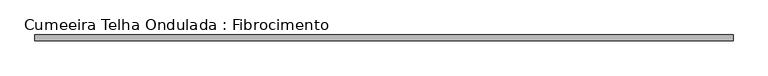
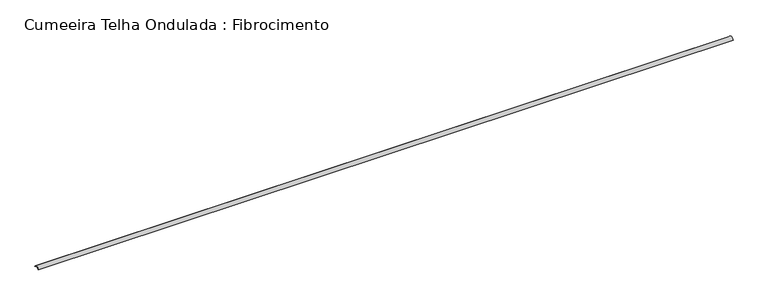
"""IFC4 building model written with IfcOpenShell, lengths in millimetres: beam geometry, Cumeeira Telha Ondulada : Fibrocimento."""

from ifc_helpers import new_model, si_unit, point, frame, frame_2d, origin, place, context, project, spatial, polyline, circle_curve, trimmed, segment, composite_curve, outline, extrude, source, transform, mapped, element, save


def cumeeira_telha_ondulada_fibrocimento_80a8fd81(model_context):
    return source(origin(), model_context, "Body", "SweptSolid", [
        extrude(outline(composite_curve([segment(polyline([(58.3970135, 42.4437972), (53.9055884, 40.2467307)]), True, "CONTINUOUS"), segment(trimmed(circle_curve(frame_2d((-1.6029865, 13.0936483)), 61.7939461), [point((53.9055884, 40.2467307))], [point((-57.1115615, 40.2467307))], True, "CARTESIAN"), True, "CONTINUOUS"), segment(polyline([(-57.1115615, 40.2467307), (-61.6029865, 42.4437972)]), True, "CONTINUOUS"), segment(trimmed(circle_curve(frame_2d((-1.6029865, 13.0936483)), 66.7939461), [point((-61.6029865, 42.4437972))], [point((58.3970135, 42.4437972))], False, "CARTESIAN"), True, "CONTINUOUS")], self_intersect=False)), frame((-7085.3584094, 0.0, 0.0), z_axis=(1.0, 0.0, 0.0), x_axis=(0.0, 1.0, 0.0)), (0.0, 0.0, 1.0), 14170.7168187),
    ])


if __name__ == "__main__":
    model = new_model("IFC4")
    model_context = context("Model", 3, world=origin())
    ifc_project = project(units=[si_unit("LENGTHUNIT", "METRE", prefix="MILLI")], contexts=[model_context])
    site = spatial("IfcSite", under=ifc_project)
    building = spatial("IfcBuilding", under=site)
    placement = place(None, origin())
    cumeeira_telha_ondulada_fibrocimento_shape = cumeeira_telha_ondulada_fibrocimento_80a8fd81(model_context)
    element("IfcBeam", 1, ObjectType="Cumeeira Telha Ondulada : Fibrocimento", at=placement, inside=building, context=model_context, shape_type="MappedRepresentation", body=[
        mapped(cumeeira_telha_ondulada_fibrocimento_shape, transform((0.0, 0.0, 0.0), x_axis=(1.0, 0.0, 0.0), y_axis=(0.0, 1.0, 0.0), z_axis=(0.0, 0.0, 1.0))),
    ])
    save(model, "model.ifc")

# Revit data of these elements
# Type "Cumeeira Telha Ondulada : Fibrocimento"
#   Cost = 5
#   Length [instance default] = 1.524 m
#   b = 0.07 m
#   h = 0.16 m
#   Structural Material = .TELHA DE FIBROCIMENTO
#   Assembly Code = ""
# Element 1 (IfcBeam, "Cumeeira Telha Ondulada : Fibrocimento")
#   Materials on its faces: ".TELHA DE FIBROCIMENTO"
# Materials
#   ".TELHA DE FIBROCIMENTO": class "CC_TELHADO", colour RGB 77 77 76, transparency 0, Description = "TELHA ONDULADA FIBROCIMENTO", Cost = 0
